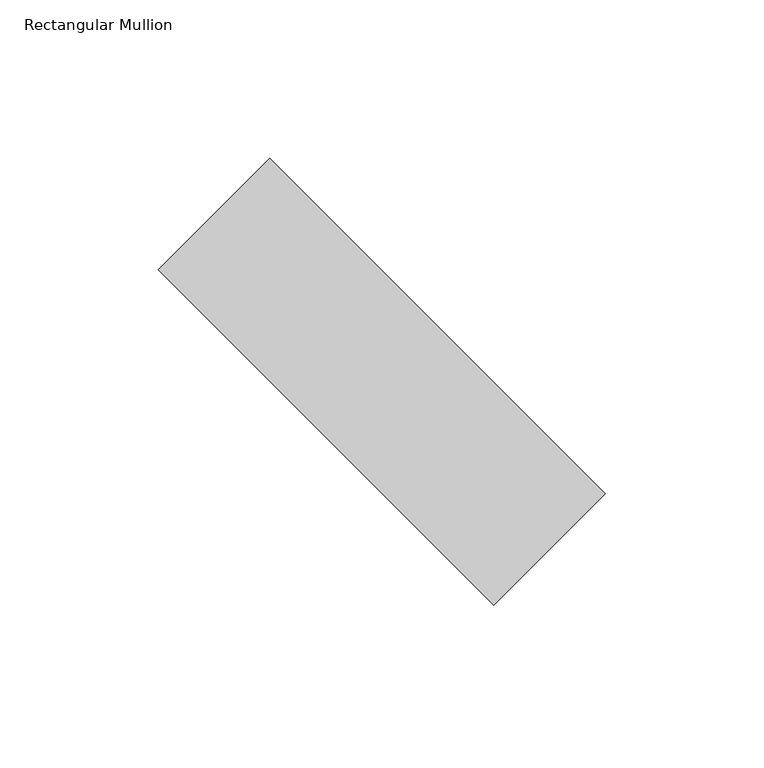
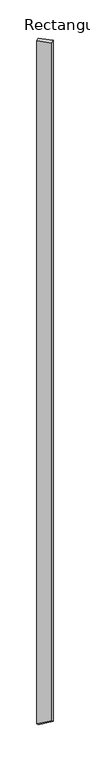
"""IFC4 building model written with IfcOpenShell, lengths in millimetres: member geometry, Rectangular Mullion : tilted mullions."""

from ifc_helpers import new_model, si_unit, origin, place, context, project, spatial, faceted_brep, source, transform, mapped, element, save


def rectangular_mullion_5aad1459(model_context):
    return source(origin(), model_context, "Body", "Brep", [
        faceted_brep([(-35.3553391, 70.7106781, 0.0), (-70.7106781, 35.3553391, 0.0), (35.3553391, -70.7106781, 0.0), (70.7106781, -35.3553391, 0.0), (-35.3553391, 70.7106781, -8054.3083391), (-70.7106781, 35.3553391, -8009.2609179), (35.3553391, -70.7106781, -7944.1719897), (70.7106781, -35.3553391, -7989.2194109)], [[[0, 1, 2, 3]], [[1, 0, 4, 5]], [[2, 1, 5, 6]], [[3, 2, 6, 7]], [[0, 3, 7, 4]], [[4, 7, 6, 5]]]),
    ])


if __name__ == "__main__":
    model = new_model("IFC4")
    model_context = context("Model", 3, world=origin())
    ifc_project = project(units=[si_unit("LENGTHUNIT", "METRE", prefix="MILLI")], contexts=[model_context])
    site = spatial("IfcSite", under=ifc_project)
    building = spatial("IfcBuilding", under=site)
    placement = place(None, origin())
    rectangular_mullion_shape = rectangular_mullion_5aad1459(model_context)
    element("IfcMember", 1, ObjectType="Rectangular Mullion : tilted mullions", at=placement, inside=building, context=model_context, shape_type="MappedRepresentation", body=[
        mapped(rectangular_mullion_shape, transform((0.0, 0.0, 0.0), x_axis=(1.0, 0.0, 0.0), y_axis=(0.0, 1.0, 0.0), z_axis=(0.0, 0.0, 1.0))),
    ])
    save(model, "model.ifc")

# Revit data of these elements
# Type "Rectangular Mullion : tilted mullions"
#   built-in parameter 1007304 = 0.492126 (stored number, unit not read)
#   built-in parameter 1007301 = 0.082021 (stored number, unit not read)
#   built-in parameter 1007300 = 0.082021 (stored number, unit not read)
# Element 1 (IfcMember, "Rectangular Mullion : tilted mullions")
#   Materials on its faces: "Aluminum"
# Materials
#   "Aluminum": class "Metal", colour RGB 244 244 244, transparency 0, Description = "Aluminum 6061", Cost = 0
